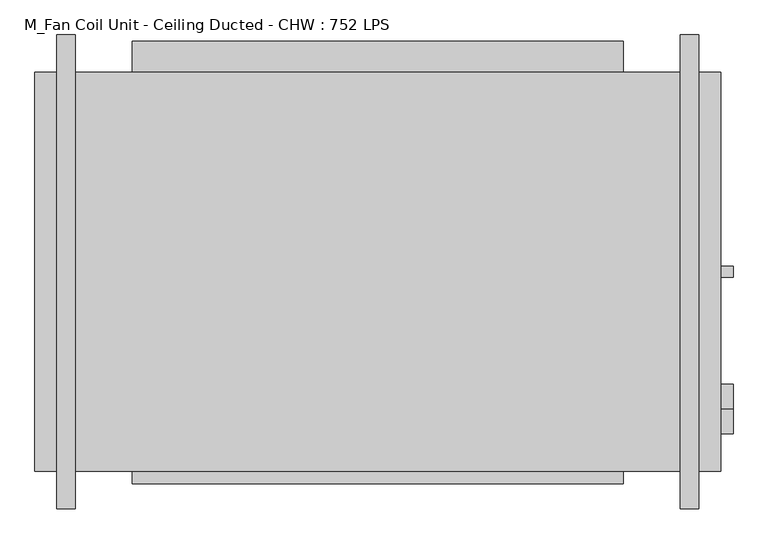
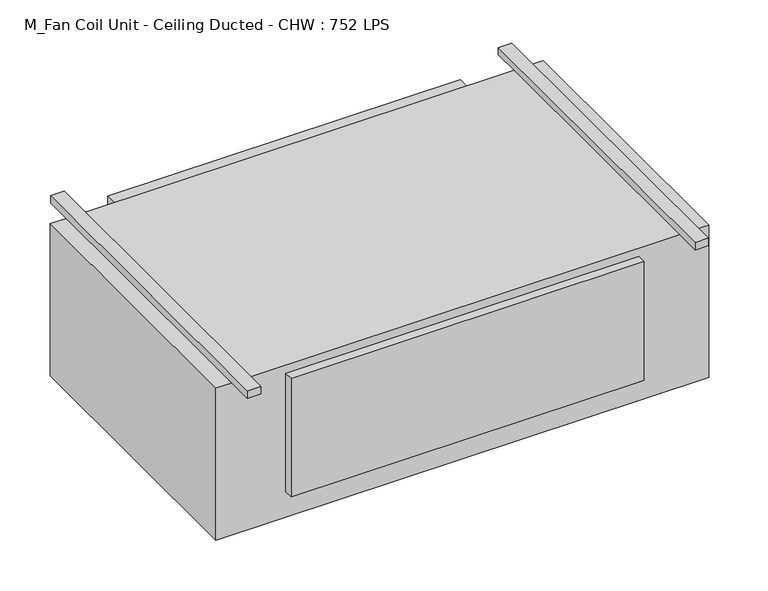
"""IFC4 building model written with IfcOpenShell, lengths in millimetres: proxy geometry, M_Fan Coil Unit - Ceiling Ducted - CHW : 752 LPS."""

from ifc_helpers import new_model, si_unit, frame, origin, place, context, project, spatial, circle_curve, source, transform, mapped, element, save
from ifc_brep_helpers import plane_surface, cylinder_surface, advanced_brep


def m_fan_coil_unit_ceiling_ducted_chw_752_lps_00c37acd(model_context):
    return source(origin(), model_context, "Body", "AdvancedBrep", [
        advanced_brep(
        [(82.55, 889.0, 479.425), (44.45, 889.0, 479.425), (44.45, -76.2, 479.425), (82.55, -76.2, 479.425), (82.55, -76.2, 457.2), (44.45, -76.2, 457.2), (44.45, 0.0, 457.2), (82.55, 0.0, 457.2), (44.45, 889.0, 457.2), (82.55, 889.0, 457.2), (82.55, 812.8, 457.2), (44.45, 812.8, 457.2), (1352.55, 889.0, 479.425), (1314.45, 889.0, 479.425), (1314.45, -76.2, 479.425), (1352.55, -76.2, 479.425), (1352.55, -76.2, 457.2), (1314.45, -76.2, 457.2), (1314.45, 0.0, 457.2), (1352.55, 0.0, 457.2), (1314.45, 889.0, 457.2), (1352.55, 889.0, 457.2), (1352.55, 812.8, 457.2), (1314.45, 812.8, 457.2), (1422.4, 127.4, 381.0), (1422.4, 177.4, 381.0), (1397.0, 127.4, 381.0), (1397.0, 177.4, 381.0), (1422.4, 76.6, 101.6), (1422.4, 126.6, 101.6), (1397.0, 76.6, 101.6), (1397.0, 126.6, 101.6), (1422.4, 395.2875, 38.1), (1422.4, 417.5125, 38.1), (1397.0, 395.2875, 38.1), (1397.0, 417.5125, 38.1), (0.0, 812.8, 457.2), (0.0, 0.0, 457.2), (1397.0, 0.0, 457.2), (1397.0, 812.8, 457.2), (1397.0, 812.8, 0.0), (1397.0, 0.0, 0.0), (0.0, 0.0, 0.0), (0.0, 812.8, 0.0), (1198.5, 812.8, 431.8), (198.5, 812.8, 431.8), (198.5, 812.8, 76.2), (1198.5, 812.8, 76.2), (198.5, 0.0, 431.8), (1198.5, 0.0, 431.8), (1198.5, 0.0, 76.2), (198.5, 0.0, 76.2), (1198.5, 876.3, 431.8), (198.5, 876.3, 431.8), (1198.5, 876.3, 76.2), (198.5, 876.3, 76.2), (198.5, -25.4, 431.8), (1198.5, -25.4, 431.8), (1198.5, -25.4, 76.2), (198.5, -25.4, 76.2)],
        [
            (0, 1),
            (1, 2),
            (2, 3),
            (3, 0),
            (4, 5),
            (5, 6),
            (6, 7),
            (7, 4),
            (8, 9),
            (9, 10),
            (10, 11),
            (11, 8),
            (0, 9),
            (8, 1),
            (11, 6),
            (5, 2),
            (4, 3),
            (7, 10),
            (12, 13),
            (13, 14),
            (14, 15),
            (15, 12),
            (16, 17),
            (17, 18),
            (18, 19),
            (19, 16),
            (20, 21),
            (21, 22),
            (22, 23),
            (23, 20),
            (12, 21),
            (20, 13),
            (23, 18),
            (17, 14),
            (16, 15),
            (19, 22),
            (24, 25, circle_curve(frame((1422.4, 152.4, 381.0), z_axis=(1.0, 0.0, 0.0), x_axis=(0.0, 1.0, 0.0)), 25.0)),
            (25, 24, circle_curve(frame((1422.4, 152.4, 381.0), z_axis=(1.0, 0.0, 0.0), x_axis=(0.0, 1.0, 0.0)), 25.0)),
            (24, 26),
            (26, 27, circle_curve(frame((1397.0, 152.4, 381.0), z_axis=(1.0, 0.0, 0.0), x_axis=(0.0, 1.0, 0.0)), 25.0)),
            (27, 25),
            (27, 26, circle_curve(frame((1397.0, 152.4, 381.0), z_axis=(1.0, 0.0, 0.0), x_axis=(0.0, 1.0, 0.0)), 25.0)),
            (28, 29, circle_curve(frame((1422.4, 101.6, 101.6), z_axis=(1.0, 0.0, 0.0), x_axis=(0.0, 1.0, 0.0)), 25.0)),
            (29, 28, circle_curve(frame((1422.4, 101.6, 101.6), z_axis=(1.0, 0.0, 0.0), x_axis=(0.0, 1.0, 0.0)), 25.0)),
            (28, 30),
            (30, 31, circle_curve(frame((1397.0, 101.6, 101.6), z_axis=(1.0, 0.0, 0.0), x_axis=(0.0, 1.0, 0.0)), 25.0)),
            (31, 29),
            (31, 30, circle_curve(frame((1397.0, 101.6, 101.6), z_axis=(1.0, 0.0, 0.0), x_axis=(0.0, 1.0, 0.0)), 25.0)),
            (32, 33, circle_curve(frame((1422.4, 406.4, 38.1), z_axis=(1.0, 0.0, 0.0), x_axis=(0.0, 1.0, 0.0)), 11.1125)),
            (33, 32, circle_curve(frame((1422.4, 406.4, 38.1), z_axis=(1.0, 0.0, 0.0), x_axis=(0.0, 1.0, 0.0)), 11.1125)),
            (32, 34),
            (34, 35, circle_curve(frame((1397.0, 406.4, 38.1), z_axis=(1.0, 0.0, 0.0), x_axis=(0.0, 1.0, 0.0)), 11.1125)),
            (35, 33),
            (35, 34, circle_curve(frame((1397.0, 406.4, 38.1), z_axis=(1.0, 0.0, 0.0), x_axis=(0.0, 1.0, 0.0)), 11.1125)),
            (36, 37),
            (37, 6),
            (11, 36),
            (38, 39),
            (39, 22),
            (19, 38),
            (23, 10),
            (7, 18),
            (40, 41),
            (41, 42),
            (42, 43),
            (43, 40),
            (43, 36),
            (39, 40),
            (44, 45),
            (45, 46),
            (46, 47),
            (47, 44),
            (42, 37),
            (41, 38),
            (48, 49),
            (49, 50),
            (50, 51),
            (51, 48),
            (52, 53),
            (53, 45),
            (44, 52),
            (54, 47),
            (46, 55),
            (55, 54),
            (52, 54),
            (55, 53),
            (48, 56),
            (56, 57),
            (57, 49),
            (50, 58),
            (58, 59),
            (59, 51),
            (59, 56),
            (58, 57),
        ],
        [
            plane_surface(frame((44.45, 889.0, 479.425), z_axis=(0.0, 0.0, 1.0), x_axis=(-1.0, 0.0, 0.0))),
            plane_surface(frame((44.45, 889.0, 457.2), z_axis=(0.0, 0.0, -1.0), x_axis=(1.0, 0.0, 0.0))),
            plane_surface(frame((82.55, 889.0, 479.425), z_axis=(0.0, 1.0, 0.0), x_axis=(0.0, 0.0, -1.0))),
            plane_surface(frame((44.45, 889.0, 479.425), z_axis=(-1.0, 0.0, 0.0), x_axis=(0.0, 0.0, -1.0))),
            plane_surface(frame((44.45, -76.2, 479.425), z_axis=(0.0, -1.0, 0.0), x_axis=(0.0, 0.0, -1.0))),
            plane_surface(frame((82.55, -76.2, 479.425), z_axis=(1.0, 0.0, 0.0), x_axis=(0.0, 0.0, -1.0))),
            plane_surface(frame((1314.45, 889.0, 479.425), z_axis=(0.0, 0.0, 1.0), x_axis=(-1.0, 0.0, 0.0))),
            plane_surface(frame((1314.45, 889.0, 457.2), z_axis=(0.0, 0.0, -1.0), x_axis=(1.0, 0.0, 0.0))),
            plane_surface(frame((1352.55, 889.0, 479.425), z_axis=(0.0, 1.0, 0.0), x_axis=(0.0, 0.0, -1.0))),
            plane_surface(frame((1314.45, 889.0, 479.425), z_axis=(-1.0, 0.0, 0.0), x_axis=(0.0, 0.0, -1.0))),
            plane_surface(frame((1314.45, -76.2, 479.425), z_axis=(0.0, -1.0, 0.0), x_axis=(0.0, 0.0, -1.0))),
            plane_surface(frame((1352.55, -76.2, 479.425), z_axis=(1.0, 0.0, 0.0), x_axis=(0.0, 0.0, -1.0))),
            plane_surface(frame((1422.4, 177.4, 381.0), z_axis=(1.0, 0.0, 0.0), x_axis=(0.0, 0.0, 1.0))),
            cylinder_surface(frame((1397.0, 152.4, 381.0), z_axis=(1.0, 0.0, 0.0), x_axis=(0.0, 1.0, 0.0)), 25.0),
            plane_surface(frame((1422.4, 126.6, 101.6), z_axis=(1.0, 0.0, 0.0), x_axis=(0.0, 0.0, 1.0))),
            cylinder_surface(frame((1397.0, 101.6, 101.6), z_axis=(1.0, 0.0, 0.0), x_axis=(0.0, 1.0, 0.0)), 25.0),
            plane_surface(frame((1422.4, 417.5125, 38.1), z_axis=(1.0, 0.0, 0.0), x_axis=(0.0, 0.0, 1.0))),
            cylinder_surface(frame((1397.0, 406.4, 38.1), z_axis=(1.0, 0.0, 0.0), x_axis=(0.0, 1.0, 0.0)), 11.1125),
            plane_surface(frame((0.0, 812.8, 457.2), z_axis=(0.0, 0.0, 1.0), x_axis=(-1.0, 0.0, 0.0))),
            plane_surface(frame((0.0, 812.8, 0.0), z_axis=(0.0, 0.0, -1.0), x_axis=(1.0, 0.0, 0.0))),
            plane_surface(frame((1397.0, 812.8, 457.2), z_axis=(0.0, 1.0, 0.0), x_axis=(0.0, 0.0, -1.0))),
            plane_surface(frame((0.0, 812.8, 457.2), z_axis=(-1.0, 0.0, 0.0), x_axis=(0.0, 0.0, -1.0))),
            plane_surface(frame((0.0, 0.0, 457.2), z_axis=(0.0, -1.0, 0.0), x_axis=(0.0, 0.0, -1.0))),
            plane_surface(frame((1397.0, 0.0, 457.2), z_axis=(1.0, 0.0, 0.0), x_axis=(0.0, 0.0, -1.0))),
            plane_surface(frame((198.5, 876.3, 431.8), z_axis=(0.0, 0.0, 1.0), x_axis=(-1.0, 0.0, 0.0))),
            plane_surface(frame((198.5, 876.3, 76.2), z_axis=(0.0, 0.0, -1.0), x_axis=(1.0, 0.0, 0.0))),
            plane_surface(frame((1198.5, 876.3, 431.8), z_axis=(0.0, 1.0, 0.0), x_axis=(0.0, 0.0, -1.0))),
            plane_surface(frame((198.5, 876.3, 431.8), z_axis=(-1.0, 0.0, 0.0), x_axis=(0.0, 0.0, -1.0))),
            plane_surface(frame((1198.5, 812.8, 431.8), z_axis=(1.0, 0.0, 0.0), x_axis=(0.0, 0.0, -1.0))),
            plane_surface(frame((198.5, 0.0, 431.8), z_axis=(0.0, 0.0, 1.0), x_axis=(-1.0, 0.0, 0.0))),
            plane_surface(frame((198.5, 0.0, 76.2), z_axis=(0.0, 0.0, -1.0), x_axis=(1.0, 0.0, 0.0))),
            plane_surface(frame((198.5, 0.0, 431.8), z_axis=(-1.0, 0.0, 0.0), x_axis=(0.0, 0.0, -1.0))),
            plane_surface(frame((198.5, -25.4, 431.8), z_axis=(0.0, -1.0, 0.0), x_axis=(0.0, 0.0, -1.0))),
            plane_surface(frame((1198.5, -25.4, 431.8), z_axis=(1.0, 0.0, 0.0), x_axis=(0.0, 0.0, -1.0))),
        ],
        [
            (0, [[1, 2, 3, 4]]),
            (1, [[5, 6, 7, 8]]),
            (1, [[9, 10, 11, 12]]),
            (2, [[-1, 13, -9, 14]]),
            (3, [[-2, -14, -12, 15, -6, 16]]),
            (4, [[-3, -16, -5, 17]]),
            (5, [[-4, -17, -8, 18, -10, -13]]),
            (6, [[19, 20, 21, 22]]),
            (7, [[23, 24, 25, 26]]),
            (7, [[27, 28, 29, 30]]),
            (8, [[-19, 31, -27, 32]]),
            (9, [[-20, -32, -30, 33, -24, 34]]),
            (10, [[-21, -34, -23, 35]]),
            (11, [[-22, -35, -26, 36, -28, -31]]),
            (12, [[37, 38]]),
            (13, [[-37, 39, 40, 41]]),
            (13, [[-38, -41, 42, -39]]),
            (14, [[43, 44]]),
            (15, [[-43, 45, 46, 47]]),
            (15, [[-44, -47, 48, -45]]),
            (16, [[49, 50]]),
            (17, [[-49, 51, 52, 53]]),
            (17, [[-50, -53, 54, -51]]),
            (18, [[55, 56, -15, 57]]),
            (18, [[58, 59, -36, 60]]),
            (18, [[61, -18, 62, -33]]),
            (19, [[63, 64, 65, 66]]),
            (20, [[-66, 67, -57, -11, -61, -29, -59, 68], [69, 70, 71, 72]]),
            (21, [[-55, -67, -65, 73]]),
            (22, [[-64, 74, -60, -25, -62, -7, -56, -73], [75, 76, 77, 78]]),
            (23, [[-58, -74, -63, -68], [-40, -42], [-46, -48], [-52, -54]]),
            (24, [[79, 80, -69, 81]]),
            (25, [[82, -71, 83, 84]]),
            (26, [[-79, 85, -84, 86]]),
            (27, [[-80, -86, -83, -70]]),
            (28, [[-81, -72, -82, -85]]),
            (29, [[87, 88, 89, -75]]),
            (30, [[90, 91, 92, -77]]),
            (31, [[-87, -78, -92, 93]]),
            (32, [[-88, -93, -91, 94]]),
            (33, [[-89, -94, -90, -76]]),
        ],
    ),
    ])


if __name__ == "__main__":
    model = new_model("IFC4")
    model_context = context("Model", 3, world=origin())
    ifc_project = project(units=[si_unit("LENGTHUNIT", "METRE", prefix="MILLI")], contexts=[model_context])
    site = spatial("IfcSite", under=ifc_project)
    building = spatial("IfcBuilding", under=site)
    placement = place(None, origin())
    m_fan_coil_unit_ceiling_ducted_chw_752_lps_shape = m_fan_coil_unit_ceiling_ducted_chw_752_lps_00c37acd(model_context)
    element("IfcBuildingElementProxy", 1, Name="M_Fan Coil Unit - Ceiling Ducted - CHW : 752 LPS", ObjectType="M_Fan Coil Unit - Ceiling Ducted - CHW : 752 LPS", at=placement, inside=building, context=model_context, shape_type="MappedRepresentation", body=[
        mapped(m_fan_coil_unit_ceiling_ducted_chw_752_lps_shape, transform((0.0, 0.0, 0.0), x_axis=(1.0, 0.0, 0.0), y_axis=(0.0, 1.0, 0.0), z_axis=(0.0, 0.0, 1.0))),
    ])
    save(model, "model.ifc")

# Revit data of these elements
# Project information
#   Project Issue Date = "Issue Date"
#   Project Status = "Project Status"
#   Client Name = "Owner"
#   Project Address = "Enter address here"
#   Project Name = "Project Name"
#   Project Number = "Project Number"
# Type "M_Fan Coil Unit - Ceiling Ducted - CHW : 752 LPS"
#   Water Pressure Drop [instance default] = 172368.9 Pa
#   Voltage = 120 V
#   Unit Length = 1397 mm
#   Total Cooling Capacity = 18961.7 W
#   Supply Water Radius = 25 mm
#   Supply Water Diameter = 50 mm
#   Supply Air Width = 1000 mm
#   Sensible Cooling Capacity = 12777.9 W
#   Return Water Radius = 25 mm
#   Return Water Diameter = 50 mm
#   Return Air Width = 1000 mm
#   Nominal Air Flow [instance default] = 755.12 L/s
#   External Static Pressure [instance default] = -74.65 Pa
#   Drain Flow [instance default] = 0.0 L/s
#   Chilled Water Flow [instance default] = 0.95 L/s
#   Apparent Load = 900 VA
#   Number of Poles = 1
#   Load Classification = Cooling
#   CFU Material = none
# Element 1 (IfcBuildingElementProxy, "M_Fan Coil Unit - Ceiling Ducted - CHW : 752 LPS")
#   Water Pressure Drop = 9652.66 Pa
#   Nominal Air Flow = 1645.0 L/s
#   External Static Pressure = 74.65 Pa
#   Chilled Water Flow = 0.25 L/s
